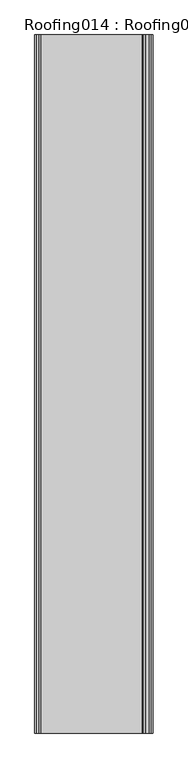
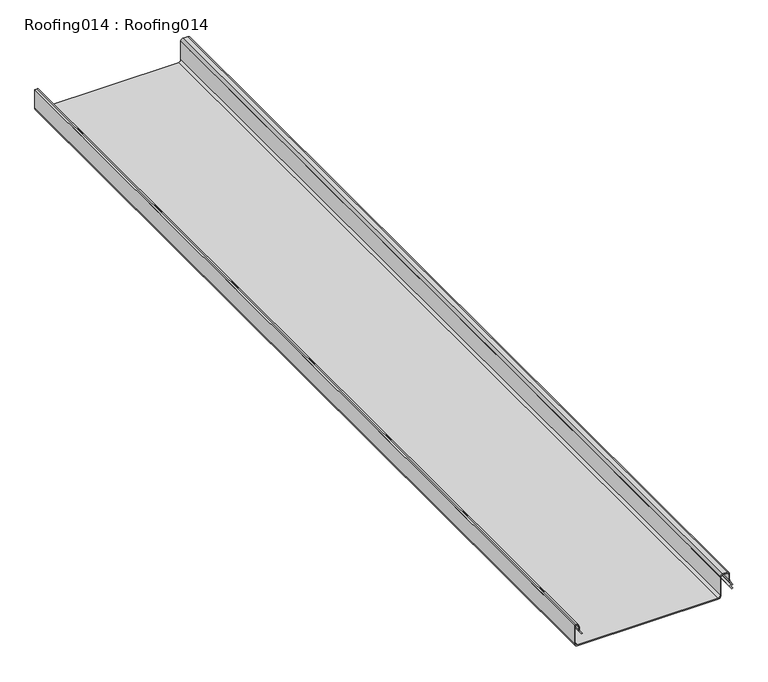
"""IFC4 building model written with IfcOpenShell, lengths in millimetres: proxy geometry, Roofing014 : Roofing014."""

from ifc_helpers import new_model, si_unit, point, frame, frame_2d, origin, place, context, project, spatial, polyline, circle_curve, trimmed, segment, composite_curve, outline, extrude, source, transform, mapped, element, save


def roofing014_roofing014_16e43a64(model_context):
    return source(origin(), model_context, "Body", "SweptSolid", [
        extrude(outline(composite_curve([segment(polyline([(43493.0126404, 17083.3738978), (43484.5384782, 17089.5215464), (43485.7128993, 17091.1404149), (43494.1870614, 17084.9927663)]), True, "CONTINUOUS"), segment(trimmed(circle_curve(frame_2d((43495.9956699, 17087.4858238)), 3.08), [point((43494.1870614, 17084.9927663))], [point((43495.9956699, 17084.4058238))], True, "CARTESIAN"), True, "CONTINUOUS"), segment(polyline([(43495.9956699, 17084.4058238), (43502.7522282, 17084.4058238)]), True, "CONTINUOUS"), segment(trimmed(circle_curve(frame_2d((43502.7522282, 17077.3258238)), 7.08), [point((43502.7522282, 17084.4058238))], [point((43509.8322282, 17077.3258238))], False, "CARTESIAN"), True, "CONTINUOUS"), segment(polyline([(43509.8322282, 17077.3258238), (43509.8322282, 17073.7310191), (43468.0950407, 17073.7310191)]), True, "CONTINUOUS"), segment(trimmed(circle_curve(frame_2d((43468.0950407, 17080.8110191)), 7.08), [point((43468.0950407, 17073.7310191))], [point((43461.0150407, 17080.8110191))], False, "CARTESIAN"), True, "CONTINUOUS"), segment(polyline([(43461.0150407, 17080.8110191), (43461.0150407, 17381.0851011)]), True, "CONTINUOUS"), segment(trimmed(circle_curve(frame_2d((43468.0950407, 17381.0851011)), 7.08), [point((43461.0150407, 17381.0851011))], [point((43468.0950407, 17388.1651011))], False, "CARTESIAN"), True, "CONTINUOUS"), segment(polyline([(43468.0950407, 17388.1651011), (43509.7084782, 17388.1651011)]), True, "CONTINUOUS"), segment(trimmed(circle_curve(frame_2d((43509.7084782, 17391.2451011)), 3.08), [point((43509.7084782, 17388.1651011))], [point((43512.7884782, 17391.2451011))], True, "CARTESIAN"), True, "CONTINUOUS"), segment(polyline([(43512.7884782, 17391.2451011), (43512.7884782, 17401.252878)]), True, "CONTINUOUS"), segment(trimmed(circle_curve(frame_2d((43509.7084782, 17401.252878)), 3.08), [point((43512.7884782, 17401.252878))], [point((43509.7084782, 17404.332878))], True, "CARTESIAN"), True, "CONTINUOUS"), segment(polyline([(43509.7084782, 17404.332878), (43496.5259041, 17404.332878)]), True, "CONTINUOUS"), segment(trimmed(circle_curve(frame_2d((43496.5259041, 17411.412878)), 7.08), [point((43496.5259041, 17404.332878))], [point((43493.0360613, 17405.2527321))], False, "CARTESIAN"), True, "CONTINUOUS"), segment(polyline([(43493.0360613, 17405.2527321), (43484.1929304, 17410.2625381), (43481.6415322, 17405.9108733), (43474.259217, 17411.1811977), (43475.4212907, 17412.8089522), (43481.0228532, 17408.8099288), (43483.4642595, 17412.9739913), (43494.0218926, 17406.9928863)]), True, "CONTINUOUS"), segment(trimmed(circle_curve(frame_2d((43496.5259041, 17411.412878)), 5.08), [point((43494.0218926, 17406.9928863))], [point((43496.5259041, 17406.332878))], True, "CARTESIAN"), True, "CONTINUOUS"), segment(polyline([(43496.5259041, 17406.332878), (43509.7084782, 17406.332878)]), True, "CONTINUOUS"), segment(trimmed(circle_curve(frame_2d((43509.7084782, 17401.252878)), 5.08), [point((43509.7084782, 17406.332878))], [point((43514.7884782, 17401.252878))], False, "CARTESIAN"), True, "CONTINUOUS"), segment(polyline([(43514.7884782, 17401.252878), (43514.7884782, 17391.2451011)]), True, "CONTINUOUS"), segment(trimmed(circle_curve(frame_2d((43509.7084782, 17391.2451011)), 5.08), [point((43514.7884782, 17391.2451011))], [point((43509.7084782, 17386.1651011))], False, "CARTESIAN"), True, "CONTINUOUS"), segment(polyline([(43509.7084782, 17386.1651011), (43468.0950407, 17386.1651011)]), True, "CONTINUOUS"), segment(trimmed(circle_curve(frame_2d((43468.0950407, 17381.0851011)), 5.08), [point((43468.0950407, 17386.1651011))], [point((43463.0150407, 17381.0851011))], True, "CARTESIAN"), True, "CONTINUOUS"), segment(polyline([(43463.0150407, 17381.0851011), (43463.0150407, 17080.8110191)]), True, "CONTINUOUS"), segment(trimmed(circle_curve(frame_2d((43468.0950407, 17080.8110191)), 5.08), [point((43463.0150407, 17080.8110191))], [point((43468.0950407, 17075.7310191))], True, "CARTESIAN"), True, "CONTINUOUS"), segment(polyline([(43468.0950407, 17075.7310191), (43507.8322282, 17075.7310191), (43507.8322282, 17077.3258238)]), True, "CONTINUOUS"), segment(trimmed(circle_curve(frame_2d((43502.7522282, 17077.3258238)), 5.08), [point((43507.8322282, 17077.3258238))], [point((43502.7522282, 17082.4058238))], True, "CARTESIAN"), True, "CONTINUOUS"), segment(polyline([(43502.7522282, 17082.4058238), (43495.9956699, 17082.4058238)]), True, "CONTINUOUS"), segment(trimmed(circle_curve(frame_2d((43495.9956699, 17087.4858238)), 5.08), [point((43495.9956699, 17082.4058238))], [point((43493.0126404, 17083.3738978))], False, "CARTESIAN"), True, "CONTINUOUS")], self_intersect=False)), frame((0.0, 7982.1507711, 0.0), z_axis=(0.0, 1.0, 0.0), x_axis=(0.0, 0.0, 1.0)), (0.0, 0.0, 1.0), 2000.0),
    ])


if __name__ == "__main__":
    model = new_model("IFC4")
    model_context = context("Model", 3, world=origin())
    ifc_project = project(units=[si_unit("LENGTHUNIT", "METRE", prefix="MILLI")], contexts=[model_context])
    site = spatial("IfcSite", under=ifc_project)
    building = spatial("IfcBuilding", under=site)
    placement = place(None, origin())
    roofing014_roofing014_shape = roofing014_roofing014_16e43a64(model_context)
    element("IfcBuildingElementProxy", 1, Name="Roofing014 : Roofing014", ObjectType="Roofing014 : Roofing014", at=placement, inside=building, context=model_context, shape_type="MappedRepresentation", body=[
        mapped(roofing014_roofing014_shape, transform((0.0, 0.0, 0.0), x_axis=(1.0, 0.0, 0.0), y_axis=(0.0, 1.0, 0.0), z_axis=(0.0, 0.0, 1.0))),
    ])
    save(model, "model.ifc")

# Revit data of these elements
# Type "Roofing014 : Roofing014"
#   NameOverride = "Roofing014"
# Element 1 (IfcBuildingElementProxy, "Roofing014 : Roofing014")
#   Materials on its faces: "STANDING SEAM METAL ROOF FOLLOW MANU. RECOMMENDED EDGE/TRANSITION DETAILS"
# Materials
#   "STANDING SEAM METAL ROOF FOLLOW MANU. RECOMMENDED EDGE/TRANSITION DETAILS": class "Unassigned", colour RGB 128 128 128, transparency 0, Cost = 0
